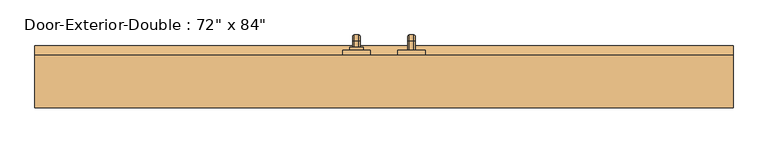
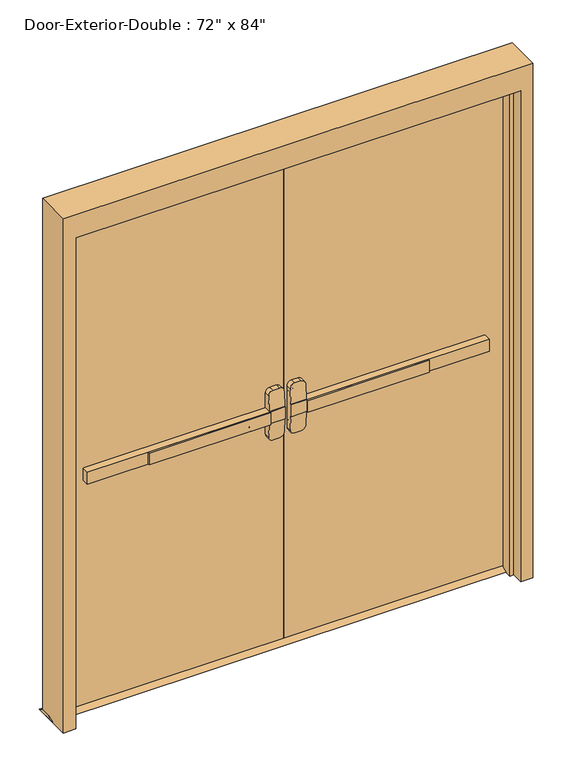
"""IFC4 building model written with IfcOpenShell, lengths in millimetres: door geometry."""

from ifc_helpers import new_model, si_unit, point, frame, frame_2d, origin, place, context, project, spatial, polyline, circle_curve, ellipse_curve, trimmed, segment, composite_curve, outline, extrude, faceted_brep, source, transform, mapped, element, save
from ifc_brep_helpers import plane_surface, cylinder_surface, revolved_surface, advanced_brep


def door_e34a14e5(model_context):
    return source(origin(), model_context, "Body", "SolidModel", [
        extrude(outline(polyline([(-575.7333333, 38.1), (-575.7333333, 44.45), (-76.2, 44.45), (-76.2, 38.1), (-575.7333333, 38.1)])), frame((0.0, 0.0, 990.6), z_axis=(0.0, 0.0, 1.0), x_axis=(1.0, 0.0, 0.0)), (0.0, 0.0, 1.0), 50.8),
        advanced_brep(
        [(-12.7, 44.45, 1041.4), (-76.2, 44.45, 1041.4), (-825.5, 44.45, 1041.4), (-825.5, 44.45, 990.6), (-76.2, 44.45, 990.6), (-12.7, 44.45, 990.6), (-825.5, 76.2, 1041.4), (-76.2, 76.2, 1041.4), (-76.2, 76.2, 1104.9), (-57.15, 76.2, 1123.95), (-31.75, 76.2, 1123.95), (-12.7, 76.2, 1104.9), (-12.7, 76.2, 927.1), (-31.75, 76.2, 908.05), (-57.15, 76.2, 908.05), (-76.2, 76.2, 927.1), (-76.2, 76.2, 990.6), (-825.5, 76.2, 990.6), (-12.7, 47.6252467, 1041.4), (-76.2, 47.6252467, 1041.4), (-12.7, 47.6252467, 990.6), (-12.7, 52.6354269, 927.1), (-12.7, 52.6354269, 1104.9), (-76.2, 47.6252467, 990.6), (-76.2, 52.6354269, 1104.9), (-76.2, 52.6354269, 927.1), (-57.15, 54.138481, 1123.95), (-31.75, 54.138481, 1123.95), (-31.75, 54.138481, 908.05), (-57.15, 54.138481, 908.05)],
        [
            (0, 1),
            (1, 2),
            (2, 3),
            (3, 4),
            (4, 5),
            (5, 0),
            (6, 7),
            (7, 8),
            (8, 9, circle_curve(frame((-57.15, 76.2, 1104.9), z_axis=(0.0, 1.0, 0.0), x_axis=(-1.0, 0.0, 0.0)), 19.05)),
            (9, 10),
            (10, 11, circle_curve(frame((-31.75, 76.2, 1104.9), z_axis=(0.0, 1.0, 0.0), x_axis=(-1.0, 0.0, 0.0)), 19.05)),
            (11, 12),
            (12, 13, circle_curve(frame((-31.75, 76.2, 927.1), z_axis=(0.0, 1.0, 0.0), x_axis=(-1.0, 0.0, 0.0)), 19.05)),
            (13, 14),
            (14, 15, circle_curve(frame((-57.15, 76.2, 927.1), z_axis=(0.0, 1.0, 0.0), x_axis=(-1.0, 0.0, 0.0)), 19.05)),
            (15, 16),
            (16, 17),
            (17, 6),
            (0, 18),
            (18, 19),
            (19, 7),
            (6, 2),
            (5, 20),
            (20, 21),
            (21, 12),
            (11, 22),
            (22, 18),
            (16, 23),
            (23, 20),
            (3, 17),
            (19, 24),
            (24, 8),
            (15, 25),
            (25, 23),
            (9, 26),
            (26, 27),
            (27, 10),
            (13, 28),
            (28, 29),
            (29, 14),
            (29, 25, ellipse_curve(frame((-57.15, 52.6354269, 927.1), z_axis=(0.0, 0.9969018152893365, 0.07865602756830282), x_axis=(0.0, -0.07865602756830208, 0.9969018152893365)), 19.1092038, 19.05)),
            (24, 26, ellipse_curve(frame((-57.15, 52.6354269, 1104.9), z_axis=(0.0, 0.9969018152893376, -0.07865602756828934), x_axis=(0.0, -0.078656027568288, -0.9969018152893377)), 19.1092038, 19.05)),
            (27, 22, ellipse_curve(frame((-31.75, 52.6354269, 1104.9), z_axis=(0.0, 0.9969018152893376, -0.07865602756828934), x_axis=(0.0, -0.078656027568288, -0.9969018152893377)), 19.1092038, 19.05)),
            (21, 28, ellipse_curve(frame((-31.75, 52.6354269, 927.1), z_axis=(0.0, 0.9969018152893365, 0.07865602756830282), x_axis=(0.0, -0.07865602756830208, 0.9969018152893365)), 19.1092038, 19.05)),
        ],
        [
            plane_surface(frame((-12.7, 44.45, 1041.4), z_axis=(0.0, -1.0, 0.0), x_axis=(1.0, 0.0, 0.0))),
            plane_surface(frame((-12.7, 76.2, 1041.4), z_axis=(0.0, 1.0, 0.0), x_axis=(-1.0, 0.0, 0.0))),
            plane_surface(frame((-825.5, 44.45, 1041.4), z_axis=(0.0, 0.0, 1.0), x_axis=(0.0, 1.0, 0.0))),
            plane_surface(frame((-12.7, 44.45, 1041.4), z_axis=(1.0, 0.0, 0.0), x_axis=(0.0, 1.0, 0.0))),
            plane_surface(frame((-12.7, 44.45, 990.6), z_axis=(0.0, 0.0, -1.0), x_axis=(0.0, 1.0, 0.0))),
            plane_surface(frame((-825.5, 44.45, 990.6), z_axis=(-1.0, 0.0, 0.0), x_axis=(0.0, 1.0, 0.0))),
            plane_surface(frame((-76.2, 47.6252467, 927.1), z_axis=(-1.0, 0.0, 0.0), x_axis=(0.0, 1.0, 0.0))),
            plane_surface(frame((-57.15, 47.6252467, 1123.95), z_axis=(0.0, 0.0, 1.0), x_axis=(0.0, 1.0, 0.0))),
            plane_surface(frame((-31.75, 47.6252467, 908.05), z_axis=(0.0, 0.0, -1.0), x_axis=(0.0, 1.0, 0.0))),
            cylinder_surface(frame((-57.15, 76.2, 927.1), z_axis=(0.0, -1.0, 0.0), x_axis=(-1.0, 0.0, 0.0)), 19.05),
            cylinder_surface(frame((-57.15, 76.2, 1104.9), z_axis=(0.0, -1.0, 0.0), x_axis=(-1.0, 0.0, 0.0)), 19.05),
            cylinder_surface(frame((-31.75, 76.2, 1104.9), z_axis=(0.0, -1.0, 0.0), x_axis=(-1.0, 0.0, 0.0)), 19.05),
            cylinder_surface(frame((-31.75, 76.2, 927.1), z_axis=(0.0, -1.0, 0.0), x_axis=(-1.0, 0.0, 0.0)), 19.05),
            plane_surface(frame((-76.2, 47.6252467, 1041.4), z_axis=(0.0, -0.9969018152893376, 0.07865602756828934), x_axis=(1.0, 0.0, 0.0))),
            plane_surface(frame((-76.2, 54.138481, 908.05), z_axis=(0.0, -0.9969018152893365, -0.07865602756830282), x_axis=(1.0, 0.0, 0.0))),
        ],
        [
            (0, [[1, 2, 3, 4, 5, 6]]),
            (1, [[7, 8, 9, 10, 11, 12, 13, 14, 15, 16, 17, 18]]),
            (2, [[-2, -1, 19, 20, 21, -7, 22]]),
            (3, [[23, 24, 25, -12, 26, 27, -19, -6]]),
            (4, [[-17, 28, 29, -23, -5, -4, 30]]),
            (5, [[-22, -18, -30, -3]]),
            (6, [[-21, 31, 32, -8]]),
            (6, [[33, 34, -28, -16]]),
            (7, [[35, 36, 37, -10]]),
            (8, [[38, 39, 40, -14]]),
            (9, [[-40, 41, -33, -15]]),
            (10, [[-32, 42, -35, -9]]),
            (11, [[-37, 43, -26, -11]]),
            (12, [[-25, 44, -38, -13]]),
            (13, [[-27, -43, -36, -42, -31, -20]]),
            (14, [[-29, -34, -41, -39, -44, -24]]),
        ],
    ),
        extrude(outline(polyline([(120.65, 12.7), (146.05, 0.0), (50.8, 0.0), (76.2, 12.7), (120.65, 12.7)])), frame((-965.2, 0.0, 0.0), z_axis=(1.0, 0.0, 0.0), x_axis=(0.0, 1.0, 0.0)), (0.0, 0.0, 1.0), 1930.4),
        extrude(outline(polyline([(575.7333333, 38.1), (76.2, 38.1), (76.2, 44.45), (575.7333333, 44.45), (575.7333333, 38.1)])), frame((0.0, 0.0, 990.6), z_axis=(0.0, 0.0, 1.0), x_axis=(1.0, 0.0, 0.0)), (0.0, 0.0, 1.0), 50.8),
        advanced_brep(
        [(12.7, 44.45, 1041.4), (12.7, 44.45, 990.6), (76.2, 44.45, 990.6), (825.5, 44.45, 990.6), (825.5, 44.45, 1041.4), (76.2, 44.45, 1041.4), (825.5, 76.2, 1041.4), (825.5, 76.2, 990.6), (76.2, 76.2, 990.6), (76.2, 76.2, 927.1), (57.15, 76.2, 908.05), (31.75, 76.2, 908.05), (12.7, 76.2, 927.1), (12.7, 76.2, 1104.9), (31.75, 76.2, 1123.95), (57.15, 76.2, 1123.95), (76.2, 76.2, 1104.9), (76.2, 76.2, 1041.4), (76.2, 47.6252467, 1041.4), (12.7, 47.6252467, 1041.4), (12.7, 52.6354269, 1104.9), (12.7, 52.6354269, 927.1), (12.7, 47.6252467, 990.6), (76.2, 47.6252467, 990.6), (76.2, 52.6354269, 927.1), (76.2, 52.6354269, 1104.9), (31.75, 54.138481, 1123.95), (57.15, 54.138481, 1123.95), (57.15, 54.138481, 908.05), (31.75, 54.138481, 908.05)],
        [
            (0, 1),
            (1, 2),
            (2, 3),
            (3, 4),
            (4, 5),
            (5, 0),
            (6, 7),
            (7, 8),
            (8, 9),
            (9, 10, circle_curve(frame((57.15, 76.2, 927.1), z_axis=(0.0, 1.0, 0.0), x_axis=(1.0, 0.0, 0.0)), 19.05)),
            (10, 11),
            (11, 12, circle_curve(frame((31.75, 76.2, 927.1), z_axis=(0.0, 1.0, 0.0), x_axis=(1.0, 0.0, 0.0)), 19.05)),
            (12, 13),
            (13, 14, circle_curve(frame((31.75, 76.2, 1104.9), z_axis=(0.0, 1.0, 0.0), x_axis=(1.0, 0.0, 0.0)), 19.05)),
            (14, 15),
            (15, 16, circle_curve(frame((57.15, 76.2, 1104.9), z_axis=(0.0, 1.0, 0.0), x_axis=(1.0, 0.0, 0.0)), 19.05)),
            (16, 17),
            (17, 6),
            (4, 6),
            (17, 18),
            (18, 19),
            (19, 0),
            (19, 20),
            (20, 13),
            (12, 21),
            (21, 22),
            (22, 1),
            (7, 3),
            (22, 23),
            (23, 8),
            (23, 24),
            (24, 9),
            (16, 25),
            (25, 18),
            (14, 26),
            (26, 27),
            (27, 15),
            (10, 28),
            (28, 29),
            (29, 11),
            (24, 28, ellipse_curve(frame((57.15, 52.6354269, 927.1), z_axis=(0.0, 0.9969018152893365, 0.07865602756830282), x_axis=(0.0, -0.07865602756830208, 0.9969018152893365)), 19.1092038, 19.05)),
            (27, 25, ellipse_curve(frame((57.15, 52.6354269, 1104.9), z_axis=(0.0, 0.9969018152893376, -0.07865602756828934), x_axis=(0.0, -0.078656027568288, -0.9969018152893377)), 19.1092038, 19.05)),
            (20, 26, ellipse_curve(frame((31.75, 52.6354269, 1104.9), z_axis=(0.0, 0.9969018152893376, -0.07865602756828934), x_axis=(0.0, -0.078656027568288, -0.9969018152893377)), 19.1092038, 19.05)),
            (29, 21, ellipse_curve(frame((31.75, 52.6354269, 927.1), z_axis=(0.0, 0.9969018152893365, 0.07865602756830282), x_axis=(0.0, -0.07865602756830208, 0.9969018152893365)), 19.1092038, 19.05)),
        ],
        [
            plane_surface(frame((12.7, 44.45, 1041.4), z_axis=(0.0, -1.0, 0.0), x_axis=(-1.0, 0.0, 0.0))),
            plane_surface(frame((12.7, 76.2, 1041.4), z_axis=(0.0, 1.0, 0.0), x_axis=(1.0, 0.0, 0.0))),
            plane_surface(frame((825.5, 44.45, 1041.4), z_axis=(0.0, 0.0, 1.0), x_axis=(0.0, 1.0, 0.0))),
            plane_surface(frame((12.7, 44.45, 1041.4), z_axis=(-1.0, 0.0, 0.0), x_axis=(0.0, 1.0, 0.0))),
            plane_surface(frame((12.7, 44.45, 990.6), z_axis=(0.0, 0.0, -1.0), x_axis=(0.0, 1.0, 0.0))),
            plane_surface(frame((825.5, 44.45, 990.6), z_axis=(1.0, 0.0, 0.0), x_axis=(0.0, 1.0, 0.0))),
            plane_surface(frame((76.2, 47.6252467, 927.1), z_axis=(1.0, 0.0, 0.0), x_axis=(0.0, 1.0, 0.0))),
            plane_surface(frame((57.15, 47.6252467, 1123.95), z_axis=(0.0, 0.0, 1.0), x_axis=(0.0, 1.0, 0.0))),
            plane_surface(frame((31.75, 47.6252467, 908.05), z_axis=(0.0, 0.0, -1.0), x_axis=(0.0, 1.0, 0.0))),
            cylinder_surface(frame((57.15, 76.2, 927.1), z_axis=(0.0, -1.0, 0.0), x_axis=(1.0, 0.0, 0.0)), 19.05),
            cylinder_surface(frame((57.15, 76.2, 1104.9), z_axis=(0.0, -1.0, 0.0), x_axis=(1.0, 0.0, 0.0)), 19.05),
            cylinder_surface(frame((31.75, 76.2, 1104.9), z_axis=(0.0, -1.0, 0.0), x_axis=(1.0, 0.0, 0.0)), 19.05),
            cylinder_surface(frame((31.75, 76.2, 927.1), z_axis=(0.0, -1.0, 0.0), x_axis=(1.0, 0.0, 0.0)), 19.05),
            plane_surface(frame((76.2, 47.6252467, 1041.4), z_axis=(0.0, -0.9969018152893376, 0.07865602756828934), x_axis=(-1.0, 0.0, 0.0))),
            plane_surface(frame((76.2, 54.138481, 908.05), z_axis=(0.0, -0.9969018152893365, -0.07865602756830282), x_axis=(-1.0, 0.0, 0.0))),
        ],
        [
            (0, [[1, 2, 3, 4, 5, 6]]),
            (1, [[7, 8, 9, 10, 11, 12, 13, 14, 15, 16, 17, 18]]),
            (2, [[19, -18, 20, 21, 22, -6, -5]]),
            (3, [[-1, -22, 23, 24, -13, 25, 26, 27]]),
            (4, [[28, -3, -2, -27, 29, 30, -8]]),
            (5, [[-4, -28, -7, -19]]),
            (6, [[-9, -30, 31, 32]]),
            (6, [[-17, 33, 34, -20]]),
            (7, [[-15, 35, 36, 37]]),
            (8, [[-11, 38, 39, 40]]),
            (9, [[-10, -32, 41, -38]]),
            (10, [[-16, -37, 42, -33]]),
            (11, [[-14, -24, 43, -35]]),
            (12, [[-12, -40, 44, -25]]),
            (13, [[-21, -34, -42, -36, -43, -23]]),
            (14, [[-26, -44, -39, -41, -31, -29]]),
        ],
    ),
        advanced_brep(
        [(66.2, 133.35, 1017.190625), (66.2, 133.35, 1014.809375), (69.771875, 133.35, 1011.2375), (82.6284594, 133.35, 1011.2375), (86.2, 133.35, 1014.8090406), (86.2, 133.35, 1017.190625), (82.628125, 133.35, 1020.7625), (69.771875, 133.35, 1020.7625), (66.2, 133.35, 887.809375), (69.771875, 133.35, 884.2375), (82.628125, 133.35, 884.2375), (86.2, 133.35, 887.809375), (86.2, 133.35, 890.1909594), (82.6284594, 133.35, 893.7625), (69.771875, 133.35, 893.7625), (66.2, 133.35, 890.190625), (66.2, 158.75, 1017.190625), (66.2, 172.640625, 1003.3), (66.2, 172.640625, 901.7), (66.2, 158.75, 887.809375), (66.2, 158.75, 890.190625), (66.2, 170.259375, 901.7), (66.2, 170.259375, 1003.3), (66.2, 158.75, 1014.809375), (69.771875, 158.75, 1011.2375), (82.6284594, 158.75, 1011.2375), (86.2, 158.75, 1014.8090406), (86.2, 170.2590406, 1003.3), (86.2, 170.2590406, 901.7), (86.2, 158.75, 890.1909594), (86.2, 158.75, 887.809375), (86.2, 172.640625, 901.7), (86.2, 172.640625, 1003.3), (86.2, 158.75, 1017.190625), (82.628125, 158.75, 1020.7625), (69.771875, 158.75, 1020.7625), (69.771875, 166.6875, 1003.3), (82.6284594, 166.6875, 1003.3), (82.628125, 176.2125, 1003.3), (69.771875, 176.2125, 1003.3), (69.771875, 166.6875, 901.7), (82.6284594, 166.6875, 901.7), (82.628125, 176.2125, 901.7), (69.771875, 176.2125, 901.7), (69.771875, 158.75, 893.7625), (82.6284594, 158.75, 893.7625), (82.628125, 158.75, 884.2375), (69.771875, 158.75, 884.2375)],
        [
            (0, 1),
            (1, 2, circle_curve(frame((69.771875, 133.35, 1014.809375), z_axis=(0.0, -1.0, 0.0), x_axis=(0.0, 0.0, 1.0)), 3.571875)),
            (2, 3),
            (3, 4, circle_curve(frame((82.6284594, 133.35, 1014.8090406), z_axis=(0.0, -1.0, 0.0), x_axis=(0.0, 0.0, 1.0)), 3.5715406)),
            (4, 5),
            (5, 6, circle_curve(frame((82.628125, 133.35, 1017.190625), z_axis=(0.0, -1.0, 0.0), x_axis=(0.0, 0.0, 1.0)), 3.571875)),
            (6, 7),
            (7, 0, circle_curve(frame((69.771875, 133.35, 1017.190625), z_axis=(0.0, -1.0, 0.0), x_axis=(0.0, 0.0, 1.0)), 3.571875)),
            (8, 9, circle_curve(frame((69.771875, 133.35, 887.809375), z_axis=(0.0, -1.0, 0.0), x_axis=(0.0, 0.0, -1.0)), 3.571875)),
            (9, 10),
            (10, 11, circle_curve(frame((82.628125, 133.35, 887.809375), z_axis=(0.0, -1.0, 0.0), x_axis=(0.0, 0.0, -1.0)), 3.571875)),
            (11, 12),
            (12, 13, circle_curve(frame((82.6284594, 133.35, 890.1909594), z_axis=(0.0, -1.0, 0.0), x_axis=(0.0, 0.0, -1.0)), 3.5715406)),
            (13, 14),
            (14, 15, circle_curve(frame((69.771875, 133.35, 890.190625), z_axis=(0.0, -1.0, 0.0), x_axis=(0.0, 0.0, -1.0)), 3.571875)),
            (15, 8),
            (0, 16),
            (16, 17, circle_curve(frame((66.2, 158.75, 1003.3), z_axis=(-1.0, 0.0, 0.0), x_axis=(0.0, 0.0, 1.0)), 13.890625)),
            (17, 18),
            (18, 19, circle_curve(frame((66.2, 158.75, 901.7), z_axis=(-1.0, 0.0, 0.0), x_axis=(0.0, 1.0, 0.0)), 13.890625)),
            (19, 8),
            (15, 20),
            (20, 21, circle_curve(frame((66.2, 158.75, 901.7), z_axis=(1.0, 0.0, 0.0), x_axis=(0.0, 1.0, 0.0)), 11.509375)),
            (21, 22),
            (22, 23, circle_curve(frame((66.2, 158.75, 1003.3), z_axis=(1.0, 0.0, 0.0), x_axis=(0.0, 0.0, 1.0)), 11.509375)),
            (23, 1),
            (23, 24, circle_curve(frame((69.771875, 158.75, 1014.809375), z_axis=(0.0, -1.0, 0.0), x_axis=(0.0, 0.0, 1.0)), 3.571875)),
            (24, 2),
            (24, 25),
            (25, 3),
            (25, 26, circle_curve(frame((82.6284594, 158.75, 1014.8090406), z_axis=(0.0, -1.0, 0.0), x_axis=(0.0, 0.0, 1.0)), 3.5715406)),
            (26, 4),
            (26, 27, circle_curve(frame((86.2, 158.75, 1003.3), z_axis=(-1.0, 0.0, 0.0), x_axis=(0.0, 0.0, 1.0)), 11.5090406)),
            (27, 28),
            (28, 29, circle_curve(frame((86.2, 158.75, 901.7), z_axis=(-1.0, 0.0, 0.0), x_axis=(0.0, 1.0, 0.0)), 11.5090406)),
            (29, 12),
            (11, 30),
            (30, 31, circle_curve(frame((86.2, 158.75, 901.7), z_axis=(1.0, 0.0, 0.0), x_axis=(0.0, 1.0, 0.0)), 13.890625)),
            (31, 32),
            (32, 33, circle_curve(frame((86.2, 158.75, 1003.3), z_axis=(1.0, 0.0, 0.0), x_axis=(0.0, 0.0, 1.0)), 13.890625)),
            (33, 5),
            (33, 34, circle_curve(frame((82.628125, 158.75, 1017.190625), z_axis=(0.0, -1.0, 0.0), x_axis=(0.0, 0.0, 1.0)), 3.571875)),
            (34, 6),
            (34, 35),
            (35, 7),
            (35, 16, circle_curve(frame((69.771875, 158.75, 1017.190625), z_axis=(0.0, -1.0, 0.0), x_axis=(0.0, 0.0, 1.0)), 3.571875)),
            (36, 24, circle_curve(frame((69.771875, 158.75, 1003.3), z_axis=(1.0, 0.0, 0.0), x_axis=(0.0, 0.0, 1.0)), 7.9375)),
            (22, 36, circle_curve(frame((69.771875, 170.259375, 1003.3), z_axis=(0.0, 0.0, 1.0), x_axis=(0.0, 1.0, 0.0)), 3.571875)),
            (37, 25, circle_curve(frame((82.6284594, 158.75, 1003.3), z_axis=(1.0, 0.0, 0.0), x_axis=(0.0, 0.0, 1.0)), 7.9375)),
            (36, 37),
            (37, 27, circle_curve(frame((82.6284594, 170.2590406, 1003.3), z_axis=(0.0, 0.0, 1.0), x_axis=(0.0, 1.0, 0.0)), 3.5715406)),
            (38, 34, circle_curve(frame((82.628125, 158.75, 1003.3), z_axis=(1.0, 0.0, 0.0), x_axis=(0.0, 0.0, 1.0)), 17.4625)),
            (32, 38, circle_curve(frame((82.628125, 172.640625, 1003.3), z_axis=(0.0, 0.0, 1.0), x_axis=(0.0, 1.0, 0.0)), 3.571875)),
            (39, 35, circle_curve(frame((69.771875, 158.75, 1003.3), z_axis=(1.0, 0.0, 0.0), x_axis=(0.0, 0.0, 1.0)), 17.4625)),
            (38, 39),
            (39, 17, circle_curve(frame((69.771875, 172.640625, 1003.3), z_axis=(0.0, 0.0, 1.0), x_axis=(0.0, 1.0, 0.0)), 3.571875)),
            (21, 40, circle_curve(frame((69.771875, 170.259375, 901.7), z_axis=(0.0, 0.0, 1.0), x_axis=(0.0, 1.0, 0.0)), 3.571875)),
            (40, 36),
            (40, 41),
            (41, 37),
            (41, 28, circle_curve(frame((82.6284594, 170.2590406, 901.7), z_axis=(0.0, 0.0, 1.0), x_axis=(0.0, 1.0, 0.0)), 3.5715406)),
            (31, 42, circle_curve(frame((82.628125, 172.640625, 901.7), z_axis=(0.0, 0.0, 1.0), x_axis=(0.0, 1.0, 0.0)), 3.571875)),
            (42, 38),
            (42, 43),
            (43, 39),
            (43, 18, circle_curve(frame((69.771875, 172.640625, 901.7), z_axis=(0.0, 0.0, 1.0), x_axis=(0.0, 1.0, 0.0)), 3.571875)),
            (44, 40, circle_curve(frame((69.771875, 158.75, 901.7), z_axis=(1.0, 0.0, 0.0), x_axis=(0.0, 1.0, 0.0)), 7.9375)),
            (20, 44, circle_curve(frame((69.771875, 158.75, 890.190625), z_axis=(0.0, 1.0, 0.0), x_axis=(0.0, 0.0, -1.0)), 3.571875)),
            (45, 41, circle_curve(frame((82.6284594, 158.75, 901.7), z_axis=(1.0, 0.0, 0.0), x_axis=(0.0, 1.0, 0.0)), 7.9375)),
            (44, 45),
            (45, 29, circle_curve(frame((82.6284594, 158.75, 890.1909594), z_axis=(0.0, 1.0, 0.0), x_axis=(0.0, 0.0, -1.0)), 3.5715406)),
            (46, 42, circle_curve(frame((82.628125, 158.75, 901.7), z_axis=(1.0, 0.0, 0.0), x_axis=(0.0, 1.0, 0.0)), 17.4625)),
            (30, 46, circle_curve(frame((82.628125, 158.75, 887.809375), z_axis=(0.0, 1.0, 0.0), x_axis=(0.0, 0.0, -1.0)), 3.571875)),
            (47, 43, circle_curve(frame((69.771875, 158.75, 901.7), z_axis=(1.0, 0.0, 0.0), x_axis=(0.0, 1.0, 0.0)), 17.4625)),
            (46, 47),
            (47, 19, circle_curve(frame((69.771875, 158.75, 887.809375), z_axis=(0.0, 1.0, 0.0), x_axis=(0.0, 0.0, -1.0)), 3.571875)),
            (14, 44),
            (13, 45),
            (10, 46),
            (9, 47),
        ],
        [
            plane_surface(frame((76.2, 133.35, 1016.0), z_axis=(0.0, -1.0, 0.0), x_axis=(1.0, 0.0, 0.0))),
            plane_surface(frame((76.2, 133.35, 889.0), z_axis=(0.0, -1.0, 0.0), x_axis=(1.0, 0.0, 0.0))),
            plane_surface(frame((66.2, 133.35, 1017.190625), z_axis=(-1.0, 0.0, 0.0), x_axis=(0.0, 1.0, 0.0))),
            cylinder_surface(frame((69.771875, 133.35, 1014.809375), z_axis=(0.0, -1.0, 0.0), x_axis=(0.0, 0.0, 1.0)), 3.571875),
            plane_surface(frame((69.771875, 133.35, 1011.2375), z_axis=(0.0, 0.0, -1.0), x_axis=(0.0, 1.0, 0.0))),
            cylinder_surface(frame((82.6284594, 133.35, 1014.8090406), z_axis=(0.0, -1.0, 0.0), x_axis=(0.0, 0.0, 1.0)), 3.5715406),
            plane_surface(frame((86.2, 133.35, 1014.8090406), z_axis=(1.0, 0.0, 0.0), x_axis=(0.0, 1.0, 0.0))),
            cylinder_surface(frame((82.628125, 133.35, 1017.190625), z_axis=(0.0, -1.0, 0.0), x_axis=(0.0, 0.0, 1.0)), 3.571875),
            plane_surface(frame((82.628125, 133.35, 1020.7625), z_axis=(0.0, 0.0, 1.0), x_axis=(0.0, 1.0, 0.0))),
            cylinder_surface(frame((69.771875, 133.35, 1017.190625), z_axis=(0.0, -1.0, 0.0), x_axis=(0.0, 0.0, 1.0)), 3.571875),
            revolved_surface(trimmed(ellipse_curve(frame((69.771875, 158.75, 1014.809375), z_axis=(0.0, -1.0, 0.0), x_axis=(0.0, 0.0, 1.0)), 3.571875, 3.571875), [point((66.2, 158.75, 1014.809375))], [point((69.771875, 158.75, 1011.2375))], True, "CARTESIAN"), (76.2, 158.75, 1003.3), (-1.0, 0.0, 0.0)),
            revolved_surface(polyline([(69.771875, 158.75, 1011.2375), (82.6284594, 158.75, 1011.2375)]), (76.2, 158.75, 1003.3), (-1.0, 0.0, 0.0)),
            revolved_surface(trimmed(ellipse_curve(frame((82.6284594, 158.75, 1014.8090406), z_axis=(0.0, -1.0, 0.0), x_axis=(0.0, 0.0, 1.0)), 3.5715406, 3.5715406), [point((82.6284594, 158.75, 1011.2375))], [point((86.2, 158.75, 1014.8090406))], True, "CARTESIAN"), (76.2, 158.75, 1003.3), (-1.0, 0.0, 0.0)),
            revolved_surface(trimmed(ellipse_curve(frame((82.628125, 158.75, 1017.190625), z_axis=(0.0, -1.0, 0.0), x_axis=(0.0, 0.0, 1.0)), 3.571875, 3.571875), [point((86.2, 158.75, 1017.190625))], [point((82.628125, 158.75, 1020.7625))], True, "CARTESIAN"), (76.2, 158.75, 1003.3), (-1.0, 0.0, 0.0)),
            cylinder_surface(frame((76.2, 158.75, 1003.3), z_axis=(-1.0, 0.0, 0.0), x_axis=(0.0, 0.0, 1.0)), 17.4625),
            revolved_surface(trimmed(ellipse_curve(frame((69.771875, 158.75, 1017.190625), z_axis=(0.0, -1.0, 0.0), x_axis=(0.0, 0.0, 1.0)), 3.571875, 3.571875), [point((69.771875, 158.75, 1020.7625))], [point((66.2, 158.75, 1017.190625))], True, "CARTESIAN"), (76.2, 158.75, 1003.3), (-1.0, 0.0, 0.0)),
            cylinder_surface(frame((69.771875, 170.259375, 1003.3), z_axis=(0.0, 0.0, 1.0), x_axis=(0.0, 1.0, 0.0)), 3.571875),
            plane_surface(frame((69.771875, 166.6875, 1003.3), z_axis=(0.0, -1.0, 0.0), x_axis=(0.0, 0.0, -1.0))),
            cylinder_surface(frame((82.6284594, 170.2590406, 1003.3), z_axis=(0.0, 0.0, 1.0), x_axis=(0.0, 1.0, 0.0)), 3.5715406),
            cylinder_surface(frame((82.628125, 172.640625, 1003.3), z_axis=(0.0, 0.0, 1.0), x_axis=(0.0, 1.0, 0.0)), 3.571875),
            plane_surface(frame((82.628125, 176.2125, 1003.3), z_axis=(0.0, 1.0, 0.0), x_axis=(0.0, 0.0, -1.0))),
            cylinder_surface(frame((69.771875, 172.640625, 1003.3), z_axis=(0.0, 0.0, 1.0), x_axis=(0.0, 1.0, 0.0)), 3.571875),
            revolved_surface(trimmed(ellipse_curve(frame((69.771875, 170.259375, 901.7), z_axis=(0.0, 0.0, 1.0), x_axis=(0.0, 1.0, 0.0)), 3.571875, 3.571875), [point((66.2, 170.259375, 901.7))], [point((69.771875, 166.6875, 901.7))], True, "CARTESIAN"), (76.2, 158.75, 901.7), (-1.0, 0.0, 0.0)),
            revolved_surface(polyline([(69.771875, 166.6875, 901.7), (82.6284594, 166.6875, 901.7)]), (76.2, 158.75, 901.7), (-1.0, 0.0, 0.0)),
            revolved_surface(trimmed(ellipse_curve(frame((82.6284594, 170.2590406, 901.7), z_axis=(0.0, 0.0, 1.0), x_axis=(0.0, 1.0, 0.0)), 3.5715406, 3.5715406), [point((82.6284594, 166.6875, 901.7))], [point((86.2, 170.2590406, 901.7))], True, "CARTESIAN"), (76.2, 158.75, 901.7), (-1.0, 0.0, 0.0)),
            revolved_surface(trimmed(ellipse_curve(frame((82.628125, 172.640625, 901.7), z_axis=(0.0, 0.0, 1.0), x_axis=(0.0, 1.0, 0.0)), 3.571875, 3.571875), [point((86.2, 172.640625, 901.7))], [point((82.628125, 176.2125, 901.7))], True, "CARTESIAN"), (76.2, 158.75, 901.7), (-1.0, 0.0, 0.0)),
            cylinder_surface(frame((76.2, 158.75, 901.7), z_axis=(-1.0, 0.0, 0.0), x_axis=(0.0, 1.0, 0.0)), 17.4625),
            revolved_surface(trimmed(ellipse_curve(frame((69.771875, 172.640625, 901.7), z_axis=(0.0, 0.0, 1.0), x_axis=(0.0, 1.0, 0.0)), 3.571875, 3.571875), [point((69.771875, 176.2125, 901.7))], [point((66.2, 172.640625, 901.7))], True, "CARTESIAN"), (76.2, 158.75, 901.7), (-1.0, 0.0, 0.0)),
            cylinder_surface(frame((69.771875, 158.75, 890.190625), z_axis=(0.0, 1.0, 0.0), x_axis=(0.0, 0.0, -1.0)), 3.571875),
            plane_surface(frame((69.771875, 158.75, 893.7625), z_axis=(0.0, 0.0, 1.0), x_axis=(0.0, -1.0, 0.0))),
            cylinder_surface(frame((82.6284594, 158.75, 890.1909594), z_axis=(0.0, 1.0, 0.0), x_axis=(0.0, 0.0, -1.0)), 3.5715406),
            cylinder_surface(frame((82.628125, 158.75, 887.809375), z_axis=(0.0, 1.0, 0.0), x_axis=(0.0, 0.0, -1.0)), 3.571875),
            plane_surface(frame((82.628125, 158.75, 884.2375), z_axis=(0.0, 0.0, -1.0), x_axis=(0.0, -1.0, 0.0))),
            cylinder_surface(frame((69.771875, 158.75, 887.809375), z_axis=(0.0, 1.0, 0.0), x_axis=(0.0, 0.0, -1.0)), 3.571875),
        ],
        [
            (0, [[1, 2, 3, 4, 5, 6, 7, 8]]),
            (1, [[9, 10, 11, 12, 13, 14, 15, 16]]),
            (2, [[-1, 17, 18, 19, 20, 21, -16, 22, 23, 24, 25, 26]]),
            (3, [[-2, -26, 27, 28]]),
            (4, [[-3, -28, 29, 30]]),
            (5, [[-4, -30, 31, 32]]),
            (6, [[-5, -32, 33, 34, 35, 36, -12, 37, 38, 39, 40, 41]]),
            (7, [[-6, -41, 42, 43]]),
            (8, [[-7, -43, 44, 45]]),
            (9, [[-8, -45, 46, -17]]),
            (10, [[47, -27, -25, 48]]),
            (11, [[49, -29, -47, 50]]),
            (12, [[-33, -31, -49, 51]]),
            (13, [[52, -42, -40, 53]]),
            (14, [[54, -44, -52, 55]]),
            (15, [[-18, -46, -54, 56]]),
            (16, [[-48, -24, 57, 58]]),
            (17, [[-50, -58, 59, 60]]),
            (18, [[-51, -60, 61, -34]]),
            (19, [[-53, -39, 62, 63]]),
            (20, [[-55, -63, 64, 65]]),
            (21, [[-56, -65, 66, -19]]),
            (22, [[67, -57, -23, 68]]),
            (23, [[69, -59, -67, 70]]),
            (24, [[-35, -61, -69, 71]]),
            (25, [[72, -62, -38, 73]]),
            (26, [[74, -64, -72, 75]]),
            (27, [[-20, -66, -74, 76]]),
            (28, [[-68, -22, -15, 77]]),
            (29, [[-70, -77, -14, 78]]),
            (30, [[-71, -78, -13, -36]]),
            (31, [[-73, -37, -11, 79]]),
            (32, [[-75, -79, -10, 80]]),
            (33, [[-76, -80, -9, -21]]),
        ],
    ),
        extrude(outline(composite_curve([segment(trimmed(circle_curve(frame_2d((1113.0338574, 76.2)), 89.3016225), [point((1193.8, 114.3))], [point((1193.8, 38.1))], False, "CARTESIAN"), True, "CONTINUOUS"), segment(polyline([(1193.8, 38.1), (838.2, 38.1)]), True, "CONTINUOUS"), segment(trimmed(circle_curve(frame_2d((918.9661426, 76.2)), 89.3016225), [point((838.2, 38.1))], [point((838.2, 114.3))], False, "CARTESIAN"), True, "CONTINUOUS"), segment(polyline([(838.2, 114.3), (1193.8, 114.3)]), True, "CONTINUOUS")], self_intersect=False)), frame((0.0, 120.65, 0.0), z_axis=(0.0, 1.0, 0.0), x_axis=(0.0, 0.0, 1.0)), (0.0, 0.0, 1.0), 12.7),
        advanced_brep(
        [(-86.2, 133.35, 1017.190625), (-86.2, 133.35, 1014.809375), (-82.628125, 133.35, 1011.2375), (-69.7715406, 133.35, 1011.2375), (-66.2, 133.35, 1014.8090406), (-66.2, 133.35, 1017.190625), (-69.771875, 133.35, 1020.7625), (-82.628125, 133.35, 1020.7625), (-86.2, 133.35, 887.809375), (-82.628125, 133.35, 884.2375), (-69.771875, 133.35, 884.2375), (-66.2, 133.35, 887.809375), (-66.2, 133.35, 890.1909594), (-69.7715406, 133.35, 893.7625), (-82.628125, 133.35, 893.7625), (-86.2, 133.35, 890.190625), (-86.2, 158.75, 1017.190625), (-86.2, 172.640625, 1003.3), (-86.2, 172.640625, 901.7), (-86.2, 158.75, 887.809375), (-86.2, 158.75, 890.190625), (-86.2, 170.259375, 901.7), (-86.2, 170.259375, 1003.3), (-86.2, 158.75, 1014.809375), (-82.628125, 158.75, 1011.2375), (-69.7715406, 158.75, 1011.2375), (-66.2, 158.75, 1014.8090406), (-66.2, 170.2590406, 1003.3), (-66.2, 170.2590406, 901.7), (-66.2, 158.75, 890.1909594), (-66.2, 158.75, 887.809375), (-66.2, 172.640625, 901.7), (-66.2, 172.640625, 1003.3), (-66.2, 158.75, 1017.190625), (-69.771875, 158.75, 1020.7625), (-82.628125, 158.75, 1020.7625), (-82.628125, 166.6875, 1003.3), (-69.7715406, 166.6875, 1003.3), (-69.771875, 176.2125, 1003.3), (-82.628125, 176.2125, 1003.3), (-82.628125, 166.6875, 901.7), (-69.7715406, 166.6875, 901.7), (-69.771875, 176.2125, 901.7), (-82.628125, 176.2125, 901.7), (-82.628125, 158.75, 893.7625), (-69.7715406, 158.75, 893.7625), (-69.771875, 158.75, 884.2375), (-82.628125, 158.75, 884.2375)],
        [
            (0, 1),
            (1, 2, circle_curve(frame((-82.628125, 133.35, 1014.809375), z_axis=(0.0, -1.0, 0.0), x_axis=(0.0, 0.0, 1.0)), 3.571875)),
            (2, 3),
            (3, 4, circle_curve(frame((-69.7715406, 133.35, 1014.8090406), z_axis=(0.0, -1.0, 0.0), x_axis=(0.0, 0.0, 1.0)), 3.5715406)),
            (4, 5),
            (5, 6, circle_curve(frame((-69.771875, 133.35, 1017.190625), z_axis=(0.0, -1.0, 0.0), x_axis=(0.0, 0.0, 1.0)), 3.571875)),
            (6, 7),
            (7, 0, circle_curve(frame((-82.628125, 133.35, 1017.190625), z_axis=(0.0, -1.0, 0.0), x_axis=(0.0, 0.0, 1.0)), 3.571875)),
            (8, 9, circle_curve(frame((-82.628125, 133.35, 887.809375), z_axis=(0.0, -1.0, 0.0), x_axis=(0.0, 0.0, -1.0)), 3.571875)),
            (9, 10),
            (10, 11, circle_curve(frame((-69.771875, 133.35, 887.809375), z_axis=(0.0, -1.0, 0.0), x_axis=(0.0, 0.0, -1.0)), 3.571875)),
            (11, 12),
            (12, 13, circle_curve(frame((-69.7715406, 133.35, 890.1909594), z_axis=(0.0, -1.0, 0.0), x_axis=(0.0, 0.0, -1.0)), 3.5715406)),
            (13, 14),
            (14, 15, circle_curve(frame((-82.628125, 133.35, 890.190625), z_axis=(0.0, -1.0, 0.0), x_axis=(0.0, 0.0, -1.0)), 3.571875)),
            (15, 8),
            (0, 16),
            (16, 17, circle_curve(frame((-86.2, 158.75, 1003.3), z_axis=(-1.0, 0.0, 0.0), x_axis=(0.0, 0.0, 1.0)), 13.890625)),
            (17, 18),
            (18, 19, circle_curve(frame((-86.2, 158.75, 901.7), z_axis=(-1.0, 0.0, 0.0), x_axis=(0.0, 1.0, 0.0)), 13.890625)),
            (19, 8),
            (15, 20),
            (20, 21, circle_curve(frame((-86.2, 158.75, 901.7), z_axis=(1.0, 0.0, 0.0), x_axis=(0.0, 1.0, 0.0)), 11.509375)),
            (21, 22),
            (22, 23, circle_curve(frame((-86.2, 158.75, 1003.3), z_axis=(1.0, 0.0, 0.0), x_axis=(0.0, 0.0, 1.0)), 11.509375)),
            (23, 1),
            (23, 24, circle_curve(frame((-82.628125, 158.75, 1014.809375), z_axis=(0.0, -1.0, 0.0), x_axis=(0.0, 0.0, 1.0)), 3.571875)),
            (24, 2),
            (24, 25),
            (25, 3),
            (25, 26, circle_curve(frame((-69.7715406, 158.75, 1014.8090406), z_axis=(0.0, -1.0, 0.0), x_axis=(0.0, 0.0, 1.0)), 3.5715406)),
            (26, 4),
            (26, 27, circle_curve(frame((-66.2, 158.75, 1003.3), z_axis=(-1.0, 0.0, 0.0), x_axis=(0.0, 0.0, 1.0)), 11.5090406)),
            (27, 28),
            (28, 29, circle_curve(frame((-66.2, 158.75, 901.7), z_axis=(-1.0, 0.0, 0.0), x_axis=(0.0, 1.0, 0.0)), 11.5090406)),
            (29, 12),
            (11, 30),
            (30, 31, circle_curve(frame((-66.2, 158.75, 901.7), z_axis=(1.0, 0.0, 0.0), x_axis=(0.0, 1.0, 0.0)), 13.890625)),
            (31, 32),
            (32, 33, circle_curve(frame((-66.2, 158.75, 1003.3), z_axis=(1.0, 0.0, 0.0), x_axis=(0.0, 0.0, 1.0)), 13.890625)),
            (33, 5),
            (33, 34, circle_curve(frame((-69.771875, 158.75, 1017.190625), z_axis=(0.0, -1.0, 0.0), x_axis=(0.0, 0.0, 1.0)), 3.571875)),
            (34, 6),
            (34, 35),
            (35, 7),
            (35, 16, circle_curve(frame((-82.628125, 158.75, 1017.190625), z_axis=(0.0, -1.0, 0.0), x_axis=(0.0, 0.0, 1.0)), 3.571875)),
            (36, 24, circle_curve(frame((-82.628125, 158.75, 1003.3), z_axis=(1.0, 0.0, 0.0), x_axis=(0.0, 0.0, 1.0)), 7.9375)),
            (22, 36, circle_curve(frame((-82.628125, 170.259375, 1003.3), z_axis=(0.0, 0.0, 1.0), x_axis=(0.0, 1.0, 0.0)), 3.571875)),
            (37, 25, circle_curve(frame((-69.7715406, 158.75, 1003.3), z_axis=(1.0, 0.0, 0.0), x_axis=(0.0, 0.0, 1.0)), 7.9375)),
            (36, 37),
            (37, 27, circle_curve(frame((-69.7715406, 170.2590406, 1003.3), z_axis=(0.0, 0.0, 1.0), x_axis=(0.0, 1.0, 0.0)), 3.5715406)),
            (38, 34, circle_curve(frame((-69.771875, 158.75, 1003.3), z_axis=(1.0, 0.0, 0.0), x_axis=(0.0, 0.0, 1.0)), 17.4625)),
            (32, 38, circle_curve(frame((-69.771875, 172.640625, 1003.3), z_axis=(0.0, 0.0, 1.0), x_axis=(0.0, 1.0, 0.0)), 3.571875)),
            (39, 35, circle_curve(frame((-82.628125, 158.75, 1003.3), z_axis=(1.0, 0.0, 0.0), x_axis=(0.0, 0.0, 1.0)), 17.4625)),
            (38, 39),
            (39, 17, circle_curve(frame((-82.628125, 172.640625, 1003.3), z_axis=(0.0, 0.0, 1.0), x_axis=(0.0, 1.0, 0.0)), 3.571875)),
            (21, 40, circle_curve(frame((-82.628125, 170.259375, 901.7), z_axis=(0.0, 0.0, 1.0), x_axis=(0.0, 1.0, 0.0)), 3.571875)),
            (40, 36),
            (40, 41),
            (41, 37),
            (41, 28, circle_curve(frame((-69.7715406, 170.2590406, 901.7), z_axis=(0.0, 0.0, 1.0), x_axis=(0.0, 1.0, 0.0)), 3.5715406)),
            (31, 42, circle_curve(frame((-69.771875, 172.640625, 901.7), z_axis=(0.0, 0.0, 1.0), x_axis=(0.0, 1.0, 0.0)), 3.571875)),
            (42, 38),
            (42, 43),
            (43, 39),
            (43, 18, circle_curve(frame((-82.628125, 172.640625, 901.7), z_axis=(0.0, 0.0, 1.0), x_axis=(0.0, 1.0, 0.0)), 3.571875)),
            (44, 40, circle_curve(frame((-82.628125, 158.75, 901.7), z_axis=(1.0, 0.0, 0.0), x_axis=(0.0, 1.0, 0.0)), 7.9375)),
            (20, 44, circle_curve(frame((-82.628125, 158.75, 890.190625), z_axis=(0.0, 1.0, 0.0), x_axis=(0.0, 0.0, -1.0)), 3.571875)),
            (45, 41, circle_curve(frame((-69.7715406, 158.75, 901.7), z_axis=(1.0, 0.0, 0.0), x_axis=(0.0, 1.0, 0.0)), 7.9375)),
            (44, 45),
            (45, 29, circle_curve(frame((-69.7715406, 158.75, 890.1909594), z_axis=(0.0, 1.0, 0.0), x_axis=(0.0, 0.0, -1.0)), 3.5715406)),
            (46, 42, circle_curve(frame((-69.771875, 158.75, 901.7), z_axis=(1.0, 0.0, 0.0), x_axis=(0.0, 1.0, 0.0)), 17.4625)),
            (30, 46, circle_curve(frame((-69.771875, 158.75, 887.809375), z_axis=(0.0, 1.0, 0.0), x_axis=(0.0, 0.0, -1.0)), 3.571875)),
            (47, 43, circle_curve(frame((-82.628125, 158.75, 901.7), z_axis=(1.0, 0.0, 0.0), x_axis=(0.0, 1.0, 0.0)), 17.4625)),
            (46, 47),
            (47, 19, circle_curve(frame((-82.628125, 158.75, 887.809375), z_axis=(0.0, 1.0, 0.0), x_axis=(0.0, 0.0, -1.0)), 3.571875)),
            (14, 44),
            (13, 45),
            (10, 46),
            (9, 47),
        ],
        [
            plane_surface(frame((-76.2, 133.35, 1016.0), z_axis=(0.0, -1.0, 0.0), x_axis=(1.0, 0.0, 0.0))),
            plane_surface(frame((-76.2, 133.35, 889.0), z_axis=(0.0, -1.0, 0.0), x_axis=(1.0, 0.0, 0.0))),
            plane_surface(frame((-86.2, 133.35, 1017.190625), z_axis=(-1.0, 0.0, 0.0), x_axis=(0.0, 1.0, 0.0))),
            cylinder_surface(frame((-82.628125, 133.35, 1014.809375), z_axis=(0.0, -1.0, 0.0), x_axis=(0.0, 0.0, 1.0)), 3.571875),
            plane_surface(frame((-82.628125, 133.35, 1011.2375), z_axis=(0.0, 0.0, -1.0), x_axis=(0.0, 1.0, 0.0))),
            cylinder_surface(frame((-69.7715406, 133.35, 1014.8090406), z_axis=(0.0, -1.0, 0.0), x_axis=(0.0, 0.0, 1.0)), 3.5715406),
            plane_surface(frame((-66.2, 133.35, 1014.8090406), z_axis=(1.0, 0.0, 0.0), x_axis=(0.0, 1.0, 0.0))),
            cylinder_surface(frame((-69.771875, 133.35, 1017.190625), z_axis=(0.0, -1.0, 0.0), x_axis=(0.0, 0.0, 1.0)), 3.571875),
            plane_surface(frame((-69.771875, 133.35, 1020.7625), z_axis=(0.0, 0.0, 1.0), x_axis=(0.0, 1.0, 0.0))),
            cylinder_surface(frame((-82.628125, 133.35, 1017.190625), z_axis=(0.0, -1.0, 0.0), x_axis=(0.0, 0.0, 1.0)), 3.571875),
            revolved_surface(trimmed(ellipse_curve(frame((-82.628125, 158.75, 1014.809375), z_axis=(0.0, -1.0, 0.0), x_axis=(0.0, 0.0, 1.0)), 3.571875, 3.571875), [point((-86.2, 158.75, 1014.809375))], [point((-82.628125, 158.75, 1011.2375))], True, "CARTESIAN"), (-76.2, 158.75, 1003.3), (-1.0, 0.0, 0.0)),
            revolved_surface(polyline([(-82.628125, 158.75, 1011.2375), (-69.7715406, 158.75, 1011.2375)]), (-76.2, 158.75, 1003.3), (-1.0, 0.0, 0.0)),
            revolved_surface(trimmed(ellipse_curve(frame((-69.7715406, 158.75, 1014.8090406), z_axis=(0.0, -1.0, 0.0), x_axis=(0.0, 0.0, 1.0)), 3.5715406, 3.5715406), [point((-69.7715406, 158.75, 1011.2375))], [point((-66.2, 158.75, 1014.8090406))], True, "CARTESIAN"), (-76.2, 158.75, 1003.3), (-1.0, 0.0, 0.0)),
            revolved_surface(trimmed(ellipse_curve(frame((-69.771875, 158.75, 1017.190625), z_axis=(0.0, -1.0, 0.0), x_axis=(0.0, 0.0, 1.0)), 3.571875, 3.571875), [point((-66.2, 158.75, 1017.190625))], [point((-69.771875, 158.75, 1020.7625))], True, "CARTESIAN"), (-76.2, 158.75, 1003.3), (-1.0, 0.0, 0.0)),
            cylinder_surface(frame((-76.2, 158.75, 1003.3), z_axis=(-1.0, 0.0, 0.0), x_axis=(0.0, 0.0, 1.0)), 17.4625),
            revolved_surface(trimmed(ellipse_curve(frame((-82.628125, 158.75, 1017.190625), z_axis=(0.0, -1.0, 0.0), x_axis=(0.0, 0.0, 1.0)), 3.571875, 3.571875), [point((-82.628125, 158.75, 1020.7625))], [point((-86.2, 158.75, 1017.190625))], True, "CARTESIAN"), (-76.2, 158.75, 1003.3), (-1.0, 0.0, 0.0)),
            cylinder_surface(frame((-82.628125, 170.259375, 1003.3), z_axis=(0.0, 0.0, 1.0), x_axis=(0.0, 1.0, 0.0)), 3.571875),
            plane_surface(frame((-82.628125, 166.6875, 1003.3), z_axis=(0.0, -1.0, 0.0), x_axis=(0.0, 0.0, -1.0))),
            cylinder_surface(frame((-69.7715406, 170.2590406, 1003.3), z_axis=(0.0, 0.0, 1.0), x_axis=(0.0, 1.0, 0.0)), 3.5715406),
            cylinder_surface(frame((-69.771875, 172.640625, 1003.3), z_axis=(0.0, 0.0, 1.0), x_axis=(0.0, 1.0, 0.0)), 3.571875),
            plane_surface(frame((-69.771875, 176.2125, 1003.3), z_axis=(0.0, 1.0, 0.0), x_axis=(0.0, 0.0, -1.0))),
            cylinder_surface(frame((-82.628125, 172.640625, 1003.3), z_axis=(0.0, 0.0, 1.0), x_axis=(0.0, 1.0, 0.0)), 3.571875),
            revolved_surface(trimmed(ellipse_curve(frame((-82.628125, 170.259375, 901.7), z_axis=(0.0, 0.0, 1.0), x_axis=(0.0, 1.0, 0.0)), 3.571875, 3.571875), [point((-86.2, 170.259375, 901.7))], [point((-82.628125, 166.6875, 901.7))], True, "CARTESIAN"), (-76.2, 158.75, 901.7), (-1.0, 0.0, 0.0)),
            revolved_surface(polyline([(-82.628125, 166.6875, 901.7), (-69.7715406, 166.6875, 901.7)]), (-76.2, 158.75, 901.7), (-1.0, 0.0, 0.0)),
            revolved_surface(trimmed(ellipse_curve(frame((-69.7715406, 170.2590406, 901.7), z_axis=(0.0, 0.0, 1.0), x_axis=(0.0, 1.0, 0.0)), 3.5715406, 3.5715406), [point((-69.7715406, 166.6875, 901.7))], [point((-66.2, 170.2590406, 901.7))], True, "CARTESIAN"), (-76.2, 158.75, 901.7), (-1.0, 0.0, 0.0)),
            revolved_surface(trimmed(ellipse_curve(frame((-69.771875, 172.640625, 901.7), z_axis=(0.0, 0.0, 1.0), x_axis=(0.0, 1.0, 0.0)), 3.571875, 3.571875), [point((-66.2, 172.640625, 901.7))], [point((-69.771875, 176.2125, 901.7))], True, "CARTESIAN"), (-76.2, 158.75, 901.7), (-1.0, 0.0, 0.0)),
            cylinder_surface(frame((-76.2, 158.75, 901.7), z_axis=(-1.0, 0.0, 0.0), x_axis=(0.0, 1.0, 0.0)), 17.4625),
            revolved_surface(trimmed(ellipse_curve(frame((-82.628125, 172.640625, 901.7), z_axis=(0.0, 0.0, 1.0), x_axis=(0.0, 1.0, 0.0)), 3.571875, 3.571875), [point((-82.628125, 176.2125, 901.7))], [point((-86.2, 172.640625, 901.7))], True, "CARTESIAN"), (-76.2, 158.75, 901.7), (-1.0, 0.0, 0.0)),
            cylinder_surface(frame((-82.628125, 158.75, 890.190625), z_axis=(0.0, 1.0, 0.0), x_axis=(0.0, 0.0, -1.0)), 3.571875),
            plane_surface(frame((-82.628125, 158.75, 893.7625), z_axis=(0.0, 0.0, 1.0), x_axis=(0.0, -1.0, 0.0))),
            cylinder_surface(frame((-69.7715406, 158.75, 890.1909594), z_axis=(0.0, 1.0, 0.0), x_axis=(0.0, 0.0, -1.0)), 3.5715406),
            cylinder_surface(frame((-69.771875, 158.75, 887.809375), z_axis=(0.0, 1.0, 0.0), x_axis=(0.0, 0.0, -1.0)), 3.571875),
            plane_surface(frame((-69.771875, 158.75, 884.2375), z_axis=(0.0, 0.0, -1.0), x_axis=(0.0, -1.0, 0.0))),
            cylinder_surface(frame((-82.628125, 158.75, 887.809375), z_axis=(0.0, 1.0, 0.0), x_axis=(0.0, 0.0, -1.0)), 3.571875),
        ],
        [
            (0, [[1, 2, 3, 4, 5, 6, 7, 8]]),
            (1, [[9, 10, 11, 12, 13, 14, 15, 16]]),
            (2, [[-1, 17, 18, 19, 20, 21, -16, 22, 23, 24, 25, 26]]),
            (3, [[-2, -26, 27, 28]]),
            (4, [[-3, -28, 29, 30]]),
            (5, [[-4, -30, 31, 32]]),
            (6, [[-5, -32, 33, 34, 35, 36, -12, 37, 38, 39, 40, 41]]),
            (7, [[-6, -41, 42, 43]]),
            (8, [[-7, -43, 44, 45]]),
            (9, [[-8, -45, 46, -17]]),
            (10, [[47, -27, -25, 48]]),
            (11, [[49, -29, -47, 50]]),
            (12, [[-33, -31, -49, 51]]),
            (13, [[52, -42, -40, 53]]),
            (14, [[54, -44, -52, 55]]),
            (15, [[-18, -46, -54, 56]]),
            (16, [[-48, -24, 57, 58]]),
            (17, [[-50, -58, 59, 60]]),
            (18, [[-51, -60, 61, -34]]),
            (19, [[-53, -39, 62, 63]]),
            (20, [[-55, -63, 64, 65]]),
            (21, [[-56, -65, 66, -19]]),
            (22, [[67, -57, -23, 68]]),
            (23, [[69, -59, -67, 70]]),
            (24, [[-35, -61, -69, 71]]),
            (25, [[72, -62, -38, 73]]),
            (26, [[74, -64, -72, 75]]),
            (27, [[-20, -66, -74, 76]]),
            (28, [[-68, -22, -15, 77]]),
            (29, [[-70, -77, -14, 78]]),
            (30, [[-71, -78, -13, -36]]),
            (31, [[-73, -37, -11, 79]]),
            (32, [[-75, -79, -10, 80]]),
            (33, [[-76, -80, -9, -21]]),
        ],
    ),
        extrude(outline(composite_curve([segment(trimmed(circle_curve(frame_2d((1117.6, -76.2)), 19.0), [point((1117.6, -95.2))], [point((1117.6, -57.2))], False, "CARTESIAN"), True, "CONTINUOUS"), segment(trimmed(circle_curve(frame_2d((1117.6, -76.2)), 19.0), [point((1117.6, -57.2))], [point((1117.6, -95.2))], False, "CARTESIAN"), True, "CONTINUOUS")], self_intersect=False)), frame((0.0, 133.35, 0.0), z_axis=(0.0, 1.0, 0.0), x_axis=(0.0, 0.0, 1.0)), (0.0, 0.0, 1.0), 8.73125),
        extrude(outline(composite_curve([segment(trimmed(circle_curve(frame_2d((1113.0338574, -76.2)), 89.3016225), [point((1193.8, -38.1))], [point((1193.8, -114.3))], False, "CARTESIAN"), True, "CONTINUOUS"), segment(polyline([(1193.8, -114.3), (838.2, -114.3)]), True, "CONTINUOUS"), segment(trimmed(circle_curve(frame_2d((918.9661426, -76.2)), 89.3016225), [point((838.2, -114.3))], [point((838.2, -38.1))], False, "CARTESIAN"), True, "CONTINUOUS"), segment(polyline([(838.2, -38.1), (1193.8, -38.1)]), True, "CONTINUOUS")], self_intersect=False)), frame((0.0, 120.65, 0.0), z_axis=(0.0, 1.0, 0.0), x_axis=(0.0, 0.0, 1.0)), (0.0, 0.0, 1.0), 12.7),
        faceted_brep([(914.4, 71.4375, 0.0), (914.4, 120.65, 0.0), (965.2, 120.65, 0.0), (965.2, -25.4, 0.0), (914.4, -25.4, 0.0), (914.4, 23.8125, 0.0), (898.525, 23.8125, 0.0), (898.525, 71.4375, 0.0), (914.4, 71.4375, 2133.6), (914.4, 120.65, 2133.6), (-914.4, 120.65, 2133.6), (-914.4, 120.65, 0.0), (-965.2, 120.65, 0.0), (-965.2, 120.65, 2235.2), (965.2, 120.65, 2235.2), (965.2, -25.4, 2235.2), (-965.2, -25.4, 2235.2), (-965.2, -25.4, 0.0), (-914.4, -25.4, 0.0), (-914.4, -25.4, 2133.6), (914.4, -25.4, 2133.6), (914.4, 23.8125, 2133.6), (-914.4, 23.8125, 2133.6), (-914.4, 23.8125, 0.0), (-898.525, 23.8125, 0.0), (-898.525, 23.8125, 2117.725), (898.525, 23.8125, 2117.725), (898.525, 71.4375, 2117.725), (-898.525, 71.4375, 2117.725), (-898.525, 71.4375, 0.0), (-914.4, 71.4375, 0.0), (-914.4, 71.4375, 2133.6)], [[[0, 1, 2, 3, 4, 5, 6, 7]], [[1, 0, 8, 9]], [[2, 1, 9, 10, 11, 12, 13, 14]], [[3, 2, 14, 15]], [[4, 3, 15, 16, 17, 18, 19, 20]], [[5, 4, 20, 21]], [[6, 5, 21, 22, 23, 24, 25, 26]], [[7, 6, 26, 27]], [[0, 7, 27, 28, 29, 30, 31, 8]], [[9, 8, 31, 10]], [[20, 19, 22, 21]], [[26, 25, 28, 27]], [[12, 11, 30, 29, 24, 23, 18, 17]], [[11, 10, 31, 30]], [[13, 12, 17, 16]], [[19, 18, 23, 22]], [[25, 24, 29, 28]], [[15, 14, 13, 16]]]),
        extrude(outline(polyline([(914.4, 76.2), (1.5875, 76.2), (1.5875, 120.65), (914.4, 120.65), (914.4, 76.2)])), frame((0.0, 0.0, 12.7), z_axis=(0.0, 0.0, 1.0), x_axis=(1.0, 0.0, 0.0)), (0.0, 0.0, 1.0), 2120.9),
        extrude(outline(polyline([(-1.5875, 76.2), (-914.4, 76.2), (-914.4, 120.65), (-1.5875, 120.65), (-1.5875, 76.2)])), frame((0.0, 0.0, 12.7), z_axis=(0.0, 0.0, 1.0), x_axis=(1.0, 0.0, 0.0)), (0.0, 0.0, 1.0), 2120.9),
    ])


if __name__ == "__main__":
    model = new_model("IFC4")
    model_context = context("Model", 3, world=origin())
    ifc_project = project(units=[si_unit("LENGTHUNIT", "METRE", prefix="MILLI")], contexts=[model_context])
    site = spatial("IfcSite", under=ifc_project)
    building = spatial("IfcBuilding", under=site)
    placement = place(None, origin())
    door_shape = door_e34a14e5(model_context)
    element("IfcDoor", 1, ObjectType="Door-Exterior-Double : 72\" x 84\"", at=placement, inside=building, context=model_context, shape_type="MappedRepresentation", body=[
        mapped(door_shape, transform((0.0, 0.0, 0.0), x_axis=(1.0, 0.0, 0.0), y_axis=(0.0, 1.0, 0.0), z_axis=(0.0, 0.0, 1.0))),
    ])
    save(model, "model.ifc")

# Revit data of these elements
# Type "Door-Exterior-Double : 72\" x 84\""
#   Type Mark = "11"
#   Assembly Code = "B2030200"
#   Analytic Construction = "Metal"
#   Threshold Length [instance default] = 6' - 4"
#   Threshold Offset [instance default] = 0' - 0 1/2"
#   Thickness = 0' - 1 3/4"
#   Thermal Resistance (R) = 0.270118 (m²·K)/W
#   Swing Angle [instance default] = 90.00°
#   Strike Height = 3' - 4"
#   SinglePanelWidth = 3' - 0"
#   Rough Width [instance default] = 6' - 4"
#   Rough Height [instance default] = 7' - 4"
#   MFOpeningHeight [instance default] = 0' - 4"
#   MFOpeningWidth [instance default] = 0' - 4"
#   Inset Calculate [instance default] = 0' - 4"
#   Masonry Inset [instance default] = 0' - 1"
#   Height = 7' - 0"
#   Width = 6' - 0"
#   Heat Transfer Coefficient (U) = 3.70223 W/(m²·K)
#   Masonry Frame Depth = 0' - 5 3/4"
#   Threshold [instance default] = yes
#   Masonry Frame [instance default] = yes
#   Function = 1
#   Dry Wall Frame [instance default] = no
#   Threshold Material = Cherry
#   Panic Bar Material = Metal - Stainless Steel
#   Panel Material = Metal - Painted - Grey
#   Frame Material = Metal - Painted - Grey
#   Exterior Pull Material = Metal - Stainless Steel
#   Visual Light Transmittance = 0
#   Solar Heat Gain Coefficient = 0
#   Wall Closure = (empty or 0)
# Element 1 (IfcDoor, "Door-Exterior-Double : 72\" x 84\"")
#   Materials on its faces: "Metal - Stainless Steel", "Metal - Painted - Grey", "Cherry"
# Materials
#   "Cherry": class "Wood", colour RGB 154 107 61, transparency 0, Description = "Prunus Serotina", Cost = 0
#   "Metal - Stainless Steel": class "Metal", colour RGB 247 247 247, transparency 0
#   "Metal - Painted - Grey": class "Paint", colour RGB 104 104 104, transparency 0
